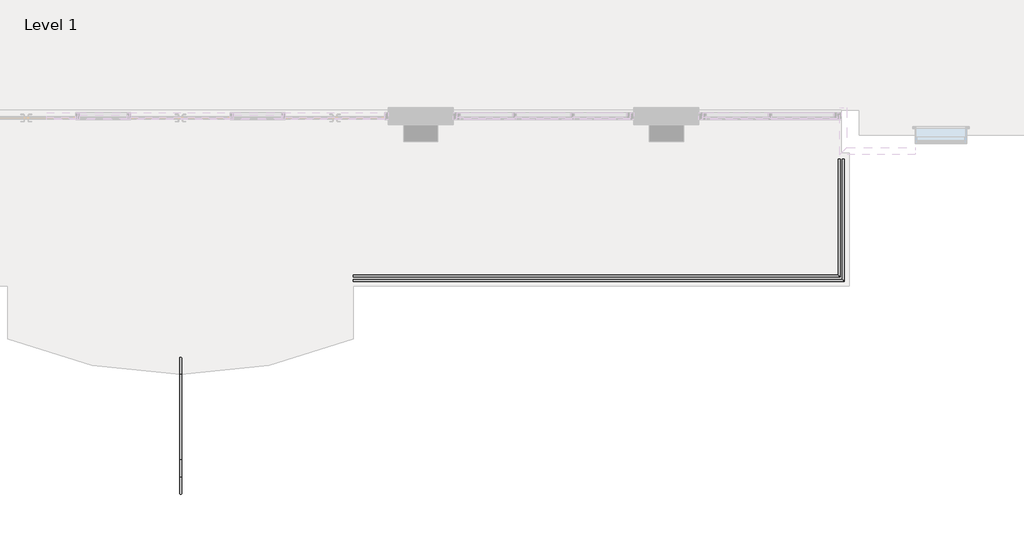
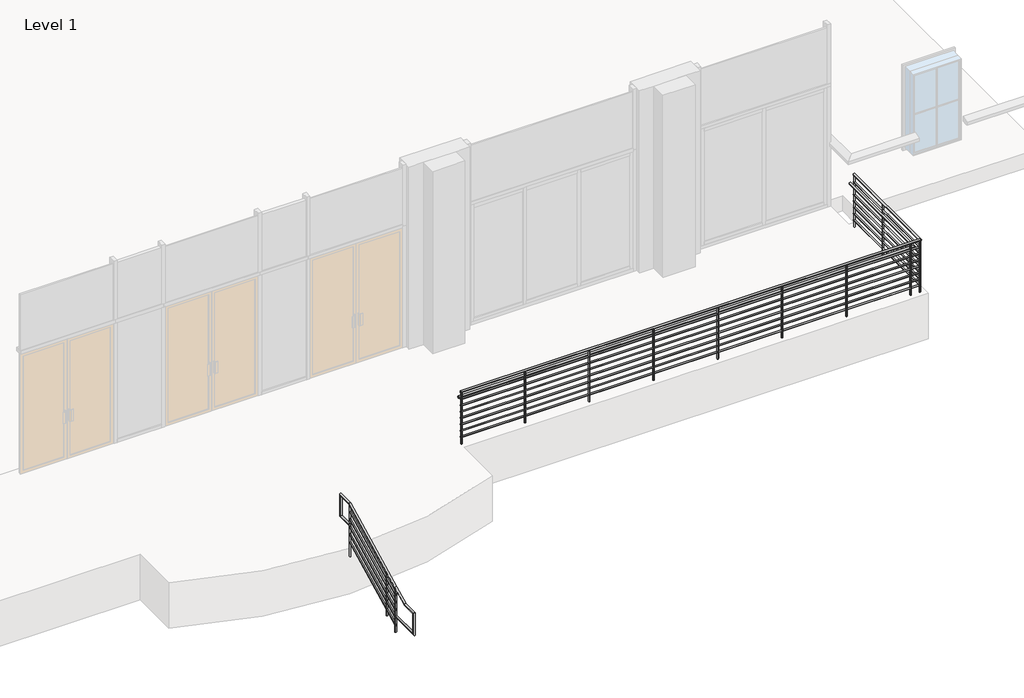
# One storey, part 3 of 5: 2 railings.
"""IFC4 building model written with IfcOpenShell, lengths in millimetres."""

import ifcopenshell
import ifcopenshell.guid

model = None  # the IFC model being written
_history = None  # IfcOwnerHistory: only IFC2X3 demands one
_inside = {}  # id of a spatial element -> (the spatial element, [elements in it])
_under = {}  # id of a project, library or spatial element -> (it, [spatial elements below it])
_declared = {}  # id of a project -> (the project, [libraries it declares])
_typed = {}  # id of a type object -> (the type object, [elements of that type])
_made_of = {}  # id of a material, layer set ... -> (it, [elements and type objects made of it])


def new_model(schema):
    """Start an empty IFC model of exactly this schema.

    Asked for "IFC4X3", IfcOpenShell would pick the latest addendum, in which some entities
    have other attributes; the version numbers below select the first issue.
    IFC2X3 requires an IfcOwnerHistory on every rooted entity: one is made here for all.
    """
    global model, _history
    if schema == "IFC4X3":
        model = ifcopenshell.file(schema_version=(4, 3, 0, 0))
    else:
        model = ifcopenshell.file(schema=schema)
    _inside.clear()
    _under.clear()
    _declared.clear()
    _typed.clear()
    _made_of.clear()
    _history = None
    if model.schema == "IFC2X3":
        org = make("IfcOrganization", Name="unknown")
        user = make(
            "IfcPersonAndOrganization",
            ThePerson=make("IfcPerson", FamilyName="unknown"),
            TheOrganization=org,
        )
        app = make(
            "IfcApplication",
            ApplicationDeveloper=org,
            Version="unknown",
            ApplicationFullName="unknown",
            ApplicationIdentifier="unknown",
        )
        _history = make(
            "IfcOwnerHistory",
            OwningUser=user,
            OwningApplication=app,
            ChangeAction="ADDED",
            CreationDate=0,
        )
    return model


def make(cls, **values):
    """One entity of the class cls with the attributes given. An attribute that is None is left unset."""
    return model.create_entity(
        cls, **{name: value for name, value in values.items() if value is not None}
    )


def rooted(cls, **values):
    """An entity with a GlobalId (a new one), such as an element, a storey or a relation."""
    return make(cls, GlobalId=ifcopenshell.guid.new(), OwnerHistory=_history, **values)


def si_unit(unit_type, name, prefix=None):
    """IfcSIUnit, for example si_unit("LENGTHUNIT", "METRE", prefix="MILLI")."""
    return make("IfcSIUnit", UnitType=unit_type, Prefix=prefix, Name=name)


def assignment(units):
    """IfcUnitAssignment: the units of a project."""
    return None if units is None else make("IfcUnitAssignment", Units=units)


def point(xyz):
    """IfcCartesianPoint."""
    return None if xyz is None else make("IfcCartesianPoint", Coordinates=xyz)


def direction(xyz):
    """IfcDirection."""
    return None if xyz is None else make("IfcDirection", DirectionRatios=xyz)


def frame(location, z_axis=None, x_axis=None):
    """IfcAxis2Placement3D, a coordinate frame: its origin and axes. An axis left out is left unset."""
    return make(
        "IfcAxis2Placement3D",
        Location=point(location),
        Axis=direction(z_axis),
        RefDirection=direction(x_axis),
    )


def frame_2d(location, x_axis=None):
    """IfcAxis2Placement2D, a coordinate frame in the plane: its origin and x axis."""
    return make(
        "IfcAxis2Placement2D", Location=point(location), RefDirection=direction(x_axis)
    )


def origin():
    """The frame at (0, 0, 0) with its axes left unset."""
    return frame((0.0, 0.0, 0.0))


def origin_with_axes():
    """The frame at (0, 0, 0) with the z axis (0, 0, 1) and the x axis (1, 0, 0) written out."""
    return frame((0.0, 0.0, 0.0), z_axis=(0.0, 0.0, 1.0), x_axis=(1.0, 0.0, 0.0))


def place(relative_to, where):
    """IfcLocalPlacement: puts the frame where relative to a parent placement (None: the world)."""
    return make(
        "IfcLocalPlacement", PlacementRelTo=relative_to, RelativePlacement=where
    )


def context(
    kind, dimensions, precision=None, world=None, true_north=None, identifier=None
):
    """IfcGeometricRepresentationContext, for example the 3D "Model" context."""
    return make(
        "IfcGeometricRepresentationContext",
        ContextIdentifier=identifier,
        ContextType=kind,
        CoordinateSpaceDimension=dimensions,
        Precision=precision,
        WorldCoordinateSystem=world,
        TrueNorth=true_north,
    )


def project(units=None, contexts=None):
    """IfcProject with its units and contexts."""
    return rooted(
        "IfcProject",
        Name="project",
        RepresentationContexts=contexts,
        UnitsInContext=assignment(units),
    )


def spatial(cls, under=None, at=None, **own):
    """A site, building, storey or space (cls), placed at a placement, below another one or the project."""
    s = rooted(cls, ObjectPlacement=at, **own)
    if under is not None:
        _under.setdefault(under.id(), (under, []))[1].append(s)
    return s


def circle_curve(where, radius):
    """IfcCircle in the frame where."""
    return make("IfcCircle", Position=where, Radius=radius)


def ellipse_curve(where, semi_axis1, semi_axis2):
    """IfcEllipse in the frame where."""
    return make(
        "IfcEllipse", Position=where, SemiAxis1=semi_axis1, SemiAxis2=semi_axis2
    )


def trimmed(basis, trim1, trim2, sense, master):
    """IfcTrimmedCurve: the piece of a basis curve between two trims."""
    return make(
        "IfcTrimmedCurve",
        BasisCurve=basis,
        Trim1=trim1,
        Trim2=trim2,
        SenseAgreement=sense,
        MasterRepresentation=master,
    )


def segment(curve, same_sense, transition):
    """IfcCompositeCurveSegment."""
    return make(
        "IfcCompositeCurveSegment",
        Transition=transition,
        SameSense=same_sense,
        ParentCurve=curve,
    )


def composite_curve(segments, self_intersect=None):
    """IfcCompositeCurve: segments joined end to end."""
    return make("IfcCompositeCurve", Segments=segments, SelfIntersect=self_intersect)


def outline(outer, holes=None, kind="AREA"):
    """IfcArbitraryClosedProfileDef: a profile drawn as a closed curve; with holes, ...WithVoids."""
    if holes is None:
        return make("IfcArbitraryClosedProfileDef", ProfileType=kind, OuterCurve=outer)
    return make(
        "IfcArbitraryProfileDefWithVoids",
        ProfileType=kind,
        OuterCurve=outer,
        InnerCurves=holes,
    )


def extrude(swept, where, along, depth):
    """IfcExtrudedAreaSolid: the profile swept, set in the frame where, extruded along a direction by depth."""
    return make(
        "IfcExtrudedAreaSolid",
        SweptArea=swept,
        Position=where,
        ExtrudedDirection=direction(along),
        Depth=depth,
    )


def shape(context_of_items, identifier, shape_type, items):
    """IfcShapeRepresentation: the items that make up one representation, for example the "Body"."""
    return make(
        "IfcShapeRepresentation",
        ContextOfItems=context_of_items,
        RepresentationIdentifier=identifier,
        RepresentationType=shape_type,
        Items=items,
    )


def made_of(thing, what):
    """Note that an element or type object is made of a material, layer set ...; save() writes the relation."""
    if what is not None:
        _made_of.setdefault(what.id(), (what, []))[1].append(thing)
    return thing


def element(
    cls,
    number,
    at=None,
    inside=None,
    cuts=None,
    type_object=None,
    material=None,
    context=None,
    identifier="Body",
    shape_type=None,
    held_by="IfcProductDefinitionShape",
    body=None,
    shapes=None,
    **own,
):
    """One element of the class cls, such as IfcWall. Its Tag is "e" and its number.

    at: its placement. inside: the storey or other place that contains it. cuts: it is an
    opening in that element (IfcRelVoidsElement). A single representation is given by context,
    identifier, shape_type and body (its items); several are given by shapes. held_by: the class
    of the entity that holds the representations. save() writes the other relations.
    """
    e = rooted(cls, Tag="e%d" % number, ObjectPlacement=at, **own)
    if body is not None:
        shapes = [shape(context, identifier, shape_type, body)]
    if shapes is not None:
        e.Representation = make(held_by, Representations=shapes)
    if inside is not None:
        _inside.setdefault(inside.id(), (inside, []))[1].append(e)
    if cuts is not None:
        rooted(
            "IfcRelVoidsElement", RelatingBuildingElement=cuts, RelatedOpeningElement=e
        )
    if type_object is not None:
        _typed.setdefault(type_object.id(), (type_object, []))[1].append(e)
    return made_of(e, material)


def aggregate(whole, parts):
    """IfcRelAggregates: a whole, such as a stair, and the parts it consists of."""
    return rooted("IfcRelAggregates", RelatingObject=whole, RelatedObjects=parts)


def save(model, path):
    """Write the relations noted so far, then the file.

    IfcRelAggregates (storeys below a building ...), IfcRelContainedInSpatialStructure (elements
    in a storey), IfcRelDefinesByType, IfcRelAssociatesMaterial and IfcRelDeclares: one each for
    every whole, place, type object, material and project.
    """
    for whole, parts in _under.values():
        aggregate(whole, parts)
    for where, things in _inside.values():
        rooted(
            "IfcRelContainedInSpatialStructure",
            RelatedElements=things,
            RelatingStructure=where,
        )
    for kind, things in _typed.values():
        rooted("IfcRelDefinesByType", RelatedObjects=things, RelatingType=kind)
    for what, things in _made_of.values():
        rooted("IfcRelAssociatesMaterial", RelatedObjects=things, RelatingMaterial=what)
    for by, libraries in _declared.values():
        rooted("IfcRelDeclares", RelatingContext=by, RelatedDefinitions=libraries)
    model.write(path)


def plane_surface(at):
    """IfcPlane: the flat surface through the origin of the frame at, square to its z axis."""
    return make("IfcPlane", Position=at)


def cylinder_surface(at, radius):
    """IfcCylindricalSurface: all points at the distance radius from the z axis of the frame at."""
    return make("IfcCylindricalSurface", Position=at, Radius=radius)


def advanced_brep(points, edges, surfaces, faces):
    """IfcAdvancedBrep: a solid bounded by faces that lie on surfaces and meet in shared edges.

    An edge is (start, end): straight between two places in points (the first is 0);
    or (start, end, curve); or (start, end, curve, False) where it runs against its curve.
    A face is (place in surfaces, loops), or (place, loops, False) where it looks against
    its surface's normal. A loop lists edges by number (the first is 1), with a minus sign
    where the edge is run from its end to its start. The first loop is the outer one.
    """
    corners = [point(p) for p in points]
    vertices = [make("IfcVertexPoint", VertexGeometry=c) for c in corners]
    made = []
    for start, end, *more in edges:
        made.append(
            make(
                "IfcEdgeCurve",
                EdgeStart=vertices[start],
                EdgeEnd=vertices[end],
                EdgeGeometry=more[0] if more else make("IfcPolyline", Points=[corners[start], corners[end]]),
                SameSense=more[1] if len(more) > 1 else True,
            )
        )
    hull = []
    for where, loops, *sense in faces:
        bounds = []
        for j, loop in enumerate(loops):
            ring = [make("IfcOrientedEdge", EdgeElement=made[abs(k) - 1], Orientation=k > 0) for k in loop]
            bounds.append(
                make(
                    "IfcFaceOuterBound" if j == 0 else "IfcFaceBound",
                    Bound=make("IfcEdgeLoop", EdgeList=ring),
                    Orientation=True,
                )
            )
        hull.append(make("IfcAdvancedFace", Bounds=bounds, FaceSurface=surfaces[where], SameSense=sense[0] if sense else True))
    return make("IfcAdvancedBrep", Outer=make("IfcClosedShell", CfsFaces=hull))


model = new_model("IFC4")

# Units and contexts
model_context = context("Model", 3, world=origin())
ifc_project = project(units=[si_unit("LENGTHUNIT", "METRE", prefix="MILLI")], contexts=[model_context])

# Site, building, storey
site = spatial("IfcSite", under=ifc_project)
building = spatial("IfcBuilding", under=site)
storey = spatial("IfcBuildingStorey", under=building, Name="Level 1", Elevation=0.0)

# Railings
placement = place(None, origin())
element("IfcRailing", 1, ObjectType="Handrail – Pipe – Bottom &Top Extension", at=placement, inside=storey, context=model_context, shape_type="AdvancedBrep", body=[
    advanced_brep(
    [(-1146.7622732, -15471.359437, -438.15), (-1184.8622732, -15471.359437, -438.15), (-1146.7622732, -16062.2278525, -438.15), (-1184.8622732, -16062.2278525, -438.15), (-1146.7622732, -16062.2278525, -19.05), (-1184.8622732, -16062.2278525, -19.05), (-1146.7622732, -15771.9807575, -19.05), (-1184.8622732, -15771.9807575, -19.05), (-1146.7622732, -15463.1584335, 135.361162), (-1184.8622732, -15463.1584335, 135.361162), (-1146.7622732, -13943.1807575, 895.35), (-1184.8622732, -13943.1807575, 895.35), (-1146.7622732, -13661.9278525, 895.35), (-1184.8622732, -13661.9278525, 895.35), (-1146.7622732, -13661.9278525, 476.25), (-1184.8622732, -13661.9278525, 476.25), (-1146.7622732, -13947.996268, 476.25), (-1184.8622732, -13947.996268, 476.25)],
    [
        (0, 1, circle_curve(frame((-1165.8122732, -15471.359437, -438.15), z_axis=(0.0, 1.0, 0.0), x_axis=(-1.0, 0.0, 0.0)), 19.05)),
        (1, 0, circle_curve(frame((-1165.8122732, -15471.359437, -438.15), z_axis=(0.0, 1.0, 0.0), x_axis=(-1.0, 0.0, 0.0)), 19.05)),
        (0, 2),
        (2, 3, ellipse_curve(frame((-1165.8122732, -16062.2278525, -438.15), z_axis=(0.0, 0.7071067811865475, -0.7071067811865475), x_axis=(0.0, 0.7071067811865476, 0.7071067811865474)), 26.9407684, 19.05)),
        (3, 1),
        (3, 2, ellipse_curve(frame((-1165.8122732, -16062.2278525, -438.15), z_axis=(0.0, 0.7071067811865475, -0.7071067811865475), x_axis=(0.0, 0.7071067811865476, 0.7071067811865474)), 26.9407684, 19.05)),
        (2, 4),
        (4, 5, ellipse_curve(frame((-1165.8122732, -16062.2278525, -19.05), z_axis=(0.0, -0.7071067811865475, -0.7071067811865475), x_axis=(0.0, 0.7071067811865474, -0.7071067811865476)), 26.9407684, 19.05)),
        (5, 3),
        (5, 4, ellipse_curve(frame((-1165.8122732, -16062.2278525, -19.05), z_axis=(0.0, -0.7071067811865475, -0.7071067811865475), x_axis=(0.0, 0.7071067811865474, -0.7071067811865476)), 26.9407684, 19.05)),
        (4, 6),
        (6, 7, ellipse_curve(frame((-1165.8122732, -15771.9807575, -19.05), z_axis=(0.0, -0.9732489894677302, -0.22975292054736124), x_axis=(0.0, -0.22975292054736096, 0.9732489894677302)), 19.573614, 19.05)),
        (7, 5),
        (7, 6, ellipse_curve(frame((-1165.8122732, -15771.9807575, -19.05), z_axis=(0.0, -0.9732489894677302, -0.22975292054736124), x_axis=(0.0, -0.22975292054736096, 0.9732489894677302)), 19.573614, 19.05)),
        (6, 8),
        (8, 9, circle_curve(frame((-1165.8122732, -15463.1584335, 135.361162), z_axis=(0.0, -0.8944271909999159, -0.44721359549995804), x_axis=(-1.0, 0.0, 0.0)), 19.05)),
        (9, 7),
        (9, 8, circle_curve(frame((-1165.8122732, -15463.1584335, 135.361162), z_axis=(0.0, -0.8944271909999159, -0.44721359549995804), x_axis=(-1.0, 0.0, 0.0)), 19.05)),
        (8, 10),
        (10, 11, ellipse_curve(frame((-1165.8122732, -13943.1807575, 895.35), z_axis=(0.0, -0.9732489894677302, -0.22975292054736132), x_axis=(0.0, 0.2297529205473615, -0.9732489894677301)), 19.573614, 19.05)),
        (11, 9),
        (11, 10, ellipse_curve(frame((-1165.8122732, -13943.1807575, 895.35), z_axis=(0.0, -0.9732489894677302, -0.22975292054736132), x_axis=(0.0, 0.2297529205473615, -0.9732489894677301)), 19.573614, 19.05)),
        (10, 12),
        (12, 13, ellipse_curve(frame((-1165.8122732, -13661.9278525, 895.35), z_axis=(0.0, -0.7071067811865476, 0.7071067811865474), x_axis=(0.0, -0.7071067811865475, -0.7071067811865475)), 26.9407684, 19.05)),
        (13, 11),
        (13, 12, ellipse_curve(frame((-1165.8122732, -13661.9278525, 895.35), z_axis=(0.0, -0.7071067811865476, 0.7071067811865474), x_axis=(0.0, -0.7071067811865475, -0.7071067811865475)), 26.9407684, 19.05)),
        (12, 14),
        (14, 15, ellipse_curve(frame((-1165.8122732, -13661.9278525, 476.25), z_axis=(0.0, 0.7071067811865474, 0.7071067811865476), x_axis=(0.0, -0.7071067811865475, 0.7071067811865475)), 26.9407684, 19.05)),
        (15, 13),
        (15, 14, ellipse_curve(frame((-1165.8122732, -13661.9278525, 476.25), z_axis=(0.0, 0.7071067811865474, 0.7071067811865476), x_axis=(0.0, -0.7071067811865475, 0.7071067811865475)), 26.9407684, 19.05)),
        (16, 17, circle_curve(frame((-1165.8122732, -13947.996268, 476.25), z_axis=(0.0, -1.0, 0.0), x_axis=(-1.0, 0.0, 0.0)), 19.05)),
        (17, 16, circle_curve(frame((-1165.8122732, -13947.996268, 476.25), z_axis=(0.0, -1.0, 0.0), x_axis=(-1.0, 0.0, 0.0)), 19.05)),
        (14, 16),
        (17, 15),
    ],
    [
        plane_surface(frame((-1165.8122732, -15471.359437, -457.2), z_axis=(0.0, 1.0, 0.0), x_axis=(0.0, 0.0, -1.0))),
        cylinder_surface(frame((-1165.8122732, -15471.359437, -438.15), z_axis=(0.0, 1.0, 0.0), x_axis=(-1.0, 0.0, 0.0)), 19.05),
        cylinder_surface(frame((-1165.8122732, -16062.2278525, -457.2), z_axis=(0.0, 0.0, -1.0), x_axis=(-1.0, 0.0, 0.0)), 19.05),
        cylinder_surface(frame((-1165.8122732, -16081.2778525, -19.05), z_axis=(0.0, -1.0, 0.0), x_axis=(-1.0, 0.0, 0.0)), 19.05),
        cylinder_surface(frame((-1165.8122732, -15767.9584335, -17.038838), z_axis=(0.0, -0.8944271909999159, -0.44721359549995804), x_axis=(-1.0, 0.0, 0.0)), 19.05),
        cylinder_surface(frame((-1165.8122732, -15463.1584335, 135.361162), z_axis=(0.0, -0.8944271909999159, -0.44721359549995804), x_axis=(-1.0, 0.0, 0.0)), 19.05),
        cylinder_surface(frame((-1165.8122732, -13947.6778525, 895.35), z_axis=(0.0, -1.0, 0.0), x_axis=(-1.0, 0.0, 0.0)), 19.05),
        cylinder_surface(frame((-1165.8122732, -13661.9278525, 914.4), z_axis=(0.0, 0.0, 1.0), x_axis=(-1.0, 0.0, 0.0)), 19.05),
        plane_surface(frame((-1165.8122732, -13947.996268, 457.2), z_axis=(0.0, -1.0, 0.0), x_axis=(0.0, 0.0, -1.0))),
        cylinder_surface(frame((-1165.8122732, -13642.8778525, 476.25), z_axis=(0.0, 1.0, 0.0), x_axis=(-1.0, 0.0, 0.0)), 19.05),
    ],
    [
        (0, [[1, 2]]),
        (1, [[-1, 3, 4, 5]]),
        (1, [[-2, -5, 6, -3]]),
        (2, [[-4, 7, 8, 9]]),
        (2, [[-6, -9, 10, -7]]),
        (3, [[-8, 11, 12, 13]]),
        (3, [[-10, -13, 14, -11]]),
        (4, [[-12, 15, 16, 17]]),
        (4, [[-14, -17, 18, -15]]),
        (5, [[-16, 19, 20, 21]]),
        (5, [[-18, -21, 22, -19]]),
        (6, [[-20, 23, 24, 25]]),
        (6, [[-22, -25, 26, -23]]),
        (7, [[-24, 27, 28, 29]]),
        (7, [[-26, -29, 30, -27]]),
        (8, [[31, 32]]),
        (9, [[-28, 33, -32, 34]]),
        (9, [[-30, -34, -31, -33]]),
    ],
),
    advanced_brep(
    [(-1153.1122732, -13947.6778525, 747.8009683), (-1178.5122732, -13947.6778525, 747.8009683), (-1153.1122732, -15471.6778525, -14.1990317), (-1178.5122732, -15471.6778525, -14.1990317)],
    [
        (0, 1, ellipse_curve(frame((-1165.8122732, -13947.6778525, 747.8009683), z_axis=(0.0, 1.0, 0.0), x_axis=(0.0, 0.0, 1.0)), 14.1990317, 12.7)),
        (1, 0, ellipse_curve(frame((-1165.8122732, -13947.6778525, 747.8009683), z_axis=(0.0, 1.0, 0.0), x_axis=(0.0, 0.0, 1.0)), 14.1990317, 12.7)),
        (2, 3, ellipse_curve(frame((-1165.8122732, -15471.6778525, -14.1990317), z_axis=(0.0, -1.0, 0.0), x_axis=(0.0, 0.0, 1.0)), 14.1990317, 12.7)),
        (3, 2, ellipse_curve(frame((-1165.8122732, -15471.6778525, -14.1990317), z_axis=(0.0, -1.0, 0.0), x_axis=(0.0, 0.0, 1.0)), 14.1990317, 12.7)),
        (0, 2),
        (3, 1),
    ],
    [
        plane_surface(frame((-1165.8122732, -13947.6778525, 762.0), z_axis=(0.0, 1.0, 0.0), x_axis=(0.0, 0.0, -1.0))),
        plane_surface(frame((-1165.8122732, -15471.6778525, 0.0), z_axis=(0.0, -1.0, 0.0), x_axis=(0.0, 0.0, -1.0))),
        cylinder_surface(frame((-1165.8122732, -13941.9982398, 750.6407747), z_axis=(0.0, 0.894427190999916, 0.447213595499958), x_axis=(-1.0, 0.0, 0.0)), 12.7),
    ],
    [
        (0, [[1, 2]]),
        (1, [[3, 4]]),
        (2, [[-1, 5, -4, 6]]),
        (2, [[-2, -6, -3, -5]]),
    ],
),
    advanced_brep(
    [(-1153.1122732, -13947.6778525, 595.4009683), (-1178.5122732, -13947.6778525, 595.4009683), (-1153.1122732, -15471.6778525, -166.5990317), (-1178.5122732, -15471.6778525, -166.5990317)],
    [
        (0, 1, ellipse_curve(frame((-1165.8122732, -13947.6778525, 595.4009683), z_axis=(0.0, 1.0, 0.0), x_axis=(0.0, 0.0, 1.0)), 14.1990317, 12.7)),
        (1, 0, ellipse_curve(frame((-1165.8122732, -13947.6778525, 595.4009683), z_axis=(0.0, 1.0, 0.0), x_axis=(0.0, 0.0, 1.0)), 14.1990317, 12.7)),
        (2, 3, ellipse_curve(frame((-1165.8122732, -15471.6778525, -166.5990317), z_axis=(0.0, -1.0, 0.0), x_axis=(0.0, 0.0, 1.0)), 14.1990317, 12.7)),
        (3, 2, ellipse_curve(frame((-1165.8122732, -15471.6778525, -166.5990317), z_axis=(0.0, -1.0, 0.0), x_axis=(0.0, 0.0, 1.0)), 14.1990317, 12.7)),
        (0, 2),
        (3, 1),
    ],
    [
        plane_surface(frame((-1165.8122732, -13947.6778525, 609.6), z_axis=(0.0, 1.0, 0.0), x_axis=(0.0, 0.0, -1.0))),
        plane_surface(frame((-1165.8122732, -15471.6778525, -152.4), z_axis=(0.0, -1.0, 0.0), x_axis=(0.0, 0.0, -1.0))),
        cylinder_surface(frame((-1165.8122732, -13941.9982398, 598.2407747), z_axis=(0.0, 0.894427190999916, 0.447213595499958), x_axis=(-1.0, 0.0, 0.0)), 12.7),
    ],
    [
        (0, [[1, 2]]),
        (1, [[3, 4]]),
        (2, [[-1, 5, -4, 6]]),
        (2, [[-2, -6, -3, -5]]),
    ],
),
    advanced_brep(
    [(-1153.1122732, -13947.6778525, 443.0009683), (-1178.5122732, -13947.6778525, 443.0009683), (-1153.1122732, -15471.6778525, -318.9990317), (-1178.5122732, -15471.6778525, -318.9990317)],
    [
        (0, 1, ellipse_curve(frame((-1165.8122732, -13947.6778525, 443.0009683), z_axis=(0.0, 1.0, 0.0), x_axis=(0.0, 0.0, 1.0)), 14.1990317, 12.7)),
        (1, 0, ellipse_curve(frame((-1165.8122732, -13947.6778525, 443.0009683), z_axis=(0.0, 1.0, 0.0), x_axis=(0.0, 0.0, 1.0)), 14.1990317, 12.7)),
        (2, 3, ellipse_curve(frame((-1165.8122732, -15471.6778525, -318.9990317), z_axis=(0.0, -1.0, 0.0), x_axis=(0.0, 0.0, 1.0)), 14.1990317, 12.7)),
        (3, 2, ellipse_curve(frame((-1165.8122732, -15471.6778525, -318.9990317), z_axis=(0.0, -1.0, 0.0), x_axis=(0.0, 0.0, 1.0)), 14.1990317, 12.7)),
        (0, 2),
        (3, 1),
    ],
    [
        plane_surface(frame((-1165.8122732, -13947.6778525, 457.2), z_axis=(0.0, 1.0, 0.0), x_axis=(0.0, 0.0, -1.0))),
        plane_surface(frame((-1165.8122732, -15471.6778525, -304.8), z_axis=(0.0, -1.0, 0.0), x_axis=(0.0, 0.0, -1.0))),
        cylinder_surface(frame((-1165.8122732, -13941.9982398, 445.8407747), z_axis=(0.0, 0.894427190999916, 0.447213595499958), x_axis=(-1.0, 0.0, 0.0)), 12.7),
    ],
    [
        (0, [[1, 2]]),
        (1, [[3, 4]]),
        (2, [[-1, 5, -4, 6]]),
        (2, [[-2, -6, -3, -5]]),
    ],
),
    advanced_brep(
    [(-1153.1122732, -13947.6778525, 290.6009683), (-1178.5122732, -13947.6778525, 290.6009683), (-1153.1122732, -15471.6778525, -471.3990317), (-1178.5122732, -15471.6778525, -471.3990317)],
    [
        (0, 1, ellipse_curve(frame((-1165.8122732, -13947.6778525, 290.6009683), z_axis=(0.0, 1.0, 0.0), x_axis=(0.0, 0.0, 1.0)), 14.1990317, 12.7)),
        (1, 0, ellipse_curve(frame((-1165.8122732, -13947.6778525, 290.6009683), z_axis=(0.0, 1.0, 0.0), x_axis=(0.0, 0.0, 1.0)), 14.1990317, 12.7)),
        (2, 3, ellipse_curve(frame((-1165.8122732, -15471.6778525, -471.3990317), z_axis=(0.0, -1.0, 0.0), x_axis=(0.0, 0.0, 1.0)), 14.1990317, 12.7)),
        (3, 2, ellipse_curve(frame((-1165.8122732, -15471.6778525, -471.3990317), z_axis=(0.0, -1.0, 0.0), x_axis=(0.0, 0.0, 1.0)), 14.1990317, 12.7)),
        (0, 2),
        (3, 1),
    ],
    [
        plane_surface(frame((-1165.8122732, -13947.6778525, 304.8), z_axis=(0.0, 1.0, 0.0), x_axis=(0.0, 0.0, -1.0))),
        plane_surface(frame((-1165.8122732, -15471.6778525, -457.2), z_axis=(0.0, -1.0, 0.0), x_axis=(0.0, 0.0, -1.0))),
        cylinder_surface(frame((-1165.8122732, -13941.9982398, 293.4407747), z_axis=(0.0, 0.894427190999916, 0.447213595499958), x_axis=(-1.0, 0.0, 0.0)), 12.7),
    ],
    [
        (0, [[1, 2]]),
        (1, [[3, 4]]),
        (2, [[-1, 5, -4, 6]]),
        (2, [[-2, -6, -3, -5]]),
    ],
),
    advanced_brep(
    [(-1153.1122732, -13947.6778525, 138.2009683), (-1178.5122732, -13947.6778525, 138.2009683), (-1153.1122732, -15471.6778525, -623.7990317), (-1178.5122732, -15471.6778525, -623.7990317)],
    [
        (0, 1, ellipse_curve(frame((-1165.8122732, -13947.6778525, 138.2009683), z_axis=(0.0, 1.0, 0.0), x_axis=(0.0, 0.0, 1.0)), 14.1990317, 12.7)),
        (1, 0, ellipse_curve(frame((-1165.8122732, -13947.6778525, 138.2009683), z_axis=(0.0, 1.0, 0.0), x_axis=(0.0, 0.0, 1.0)), 14.1990317, 12.7)),
        (2, 3, ellipse_curve(frame((-1165.8122732, -15471.6778525, -623.7990317), z_axis=(0.0, -1.0, 0.0), x_axis=(0.0, 0.0, 1.0)), 14.1990317, 12.7)),
        (3, 2, ellipse_curve(frame((-1165.8122732, -15471.6778525, -623.7990317), z_axis=(0.0, -1.0, 0.0), x_axis=(0.0, 0.0, 1.0)), 14.1990317, 12.7)),
        (0, 2),
        (3, 1),
    ],
    [
        plane_surface(frame((-1165.8122732, -13947.6778525, 152.4), z_axis=(0.0, 1.0, 0.0), x_axis=(0.0, 0.0, -1.0))),
        plane_surface(frame((-1165.8122732, -15471.6778525, -609.6), z_axis=(0.0, -1.0, 0.0), x_axis=(0.0, 0.0, -1.0))),
        cylinder_surface(frame((-1165.8122732, -13941.9982398, 141.0407747), z_axis=(0.0, 0.894427190999916, 0.447213595499958), x_axis=(-1.0, 0.0, 0.0)), 12.7),
    ],
    [
        (0, [[1, 2]]),
        (1, [[3, 4]]),
        (2, [[-1, 5, -4, 6]]),
        (2, [[-2, -6, -3, -5]]),
    ],
),
    advanced_brep(
    [(-1178.5122732, -15166.8778525, 262.202905), (-1178.5122732, -15166.8778525, -609.6), (-1153.1122732, -15166.8778525, -609.6), (-1153.1122732, -15166.8778525, 262.202905)],
    [
        (0, 1),
        (1, 2, circle_curve(frame((-1165.8122732, -15166.8778525, -609.6), z_axis=(0.0, 0.0, 1.0), x_axis=(1.0, 0.0, 0.0)), 12.7)),
        (2, 3),
        (3, 0, ellipse_curve(frame((-1165.8122732, -15166.8778525, 262.202905), z_axis=(0.0, 0.4472135954999566, -0.8944271909999165), x_axis=(0.0, 0.8944271909999165, 0.4472135954999567)), 14.1990317, 12.7)),
        (0, 3, ellipse_curve(frame((-1165.8122732, -15166.8778525, 262.202905), z_axis=(0.0, 0.4472135954999566, -0.8944271909999165), x_axis=(0.0, 0.8944271909999165, 0.4472135954999567)), 14.1990317, 12.7)),
        (2, 1, circle_curve(frame((-1165.8122732, -15166.8778525, -609.6), z_axis=(0.0, 0.0, 1.0), x_axis=(1.0, 0.0, 0.0)), 12.7)),
    ],
    [
        cylinder_surface(frame((-1165.8122732, -15166.8778525, -838.2), z_axis=(0.0, 0.0, 1.0), x_axis=(1.0, 0.0, 0.0)), 12.7),
        plane_surface(frame((-1140.4122732, -15192.2778525, 249.502905), z_axis=(0.0, -0.4472135954999566, 0.8944271909999165), x_axis=(-1.0, 0.0, 0.0))),
        plane_surface(frame((-1140.4122732, -15141.4778525, -609.6), z_axis=(0.0, 0.0, -1.0), x_axis=(-1.0, 0.0, 0.0))),
    ],
    [
        (0, [[1, 2, 3, 4]]),
        (0, [[-1, 5, -3, 6]]),
        (1, [[-4, -5]]),
        (2, [[-2, -6]]),
    ],
),
    advanced_brep(
    [(-1178.5122732, -15458.9778525, 116.152905), (-1178.5122732, -15458.9778525, -762.0), (-1153.1122732, -15458.9778525, -762.0), (-1153.1122732, -15458.9778525, 116.152905)],
    [
        (0, 1),
        (1, 2, circle_curve(frame((-1165.8122732, -15458.9778525, -762.0), z_axis=(0.0, 0.0, 1.0), x_axis=(1.0, 0.0, 0.0)), 12.7)),
        (2, 3),
        (3, 0, ellipse_curve(frame((-1165.8122732, -15458.9778525, 116.152905), z_axis=(0.0, 0.4472135954999566, -0.8944271909999165), x_axis=(0.0, 0.8944271909999165, 0.4472135954999567)), 14.1990317, 12.7)),
        (0, 3, ellipse_curve(frame((-1165.8122732, -15458.9778525, 116.152905), z_axis=(0.0, 0.4472135954999566, -0.8944271909999165), x_axis=(0.0, 0.8944271909999165, 0.4472135954999567)), 14.1990317, 12.7)),
        (2, 1, circle_curve(frame((-1165.8122732, -15458.9778525, -762.0), z_axis=(0.0, 0.0, 1.0), x_axis=(1.0, 0.0, 0.0)), 12.7)),
    ],
    [
        cylinder_surface(frame((-1165.8122732, -15458.9778525, -990.6), z_axis=(0.0, 0.0, 1.0), x_axis=(1.0, 0.0, 0.0)), 12.7),
        plane_surface(frame((-1140.4122732, -15484.3778525, 103.452905), z_axis=(0.0, -0.4472135954999566, 0.8944271909999165), x_axis=(-1.0, 0.0, 0.0))),
        plane_surface(frame((-1140.4122732, -15433.5778525, -762.0), z_axis=(0.0, 0.0, -1.0), x_axis=(-1.0, 0.0, 0.0))),
    ],
    [
        (0, [[1, 2, 3, 4]]),
        (0, [[-1, 5, -3, 6]]),
        (1, [[-4, -5]]),
        (2, [[-2, -6]]),
    ],
),
    advanced_brep(
    [(-1178.5122732, -13960.3778525, 865.452905), (-1178.5122732, -13960.3778525, -152.4), (-1153.1122732, -13960.3778525, -152.4), (-1153.1122732, -13960.3778525, 865.452905)],
    [
        (0, 1),
        (1, 2, circle_curve(frame((-1165.8122732, -13960.3778525, -152.4), z_axis=(0.0, 0.0, 1.0), x_axis=(1.0, 0.0, 0.0)), 12.7)),
        (2, 3),
        (3, 0, ellipse_curve(frame((-1165.8122732, -13960.3778525, 865.452905), z_axis=(0.0, 0.4472135954999566, -0.8944271909999165), x_axis=(0.0, 0.8944271909999165, 0.4472135954999567)), 14.1990317, 12.7)),
        (0, 3, ellipse_curve(frame((-1165.8122732, -13960.3778525, 865.452905), z_axis=(0.0, 0.4472135954999566, -0.8944271909999165), x_axis=(0.0, 0.8944271909999165, 0.4472135954999567)), 14.1990317, 12.7)),
        (2, 1, circle_curve(frame((-1165.8122732, -13960.3778525, -152.4), z_axis=(0.0, 0.0, 1.0), x_axis=(1.0, 0.0, 0.0)), 12.7)),
    ],
    [
        cylinder_surface(frame((-1165.8122732, -13960.3778525, -381.0), z_axis=(0.0, 0.0, 1.0), x_axis=(1.0, 0.0, 0.0)), 12.7),
        plane_surface(frame((-1140.4122732, -13985.7778525, 852.752905), z_axis=(0.0, -0.4472135954999566, 0.8944271909999165), x_axis=(-1.0, 0.0, 0.0))),
        plane_surface(frame((-1140.4122732, -13934.9778525, -152.4), z_axis=(0.0, 0.0, -1.0), x_axis=(-1.0, 0.0, 0.0))),
    ],
    [
        (0, [[1, 2, 3, 4]]),
        (0, [[-1, 5, -3, 6]]),
        (1, [[-4, -5]]),
        (2, [[-2, -6]]),
    ],
),
])
element("IfcRailing", 2, ObjectType="Guardrail - Pipe", at=placement, inside=storey, context=model_context, shape_type="SolidModel", body=[
    advanced_brep(
    [(1903.9547354, -12217.7608439, 895.35), (1903.9547354, -12179.6608439, 895.35), (10558.224655, -12217.7608439, 895.35), (10520.124655, -12179.6608439, 895.35), (10558.224655, -10114.0984696, 895.35), (10520.124655, -10114.0984696, 895.35)],
    [
        (0, 1, circle_curve(frame((1903.9547354, -12198.7108439, 895.35), z_axis=(-1.0, 0.0, 0.0), x_axis=(0.0, 1.0, 0.0)), 19.05)),
        (1, 0, circle_curve(frame((1903.9547354, -12198.7108439, 895.35), z_axis=(-1.0, 0.0, 0.0), x_axis=(0.0, 1.0, 0.0)), 19.05)),
        (0, 2),
        (2, 3, ellipse_curve(frame((10539.174655, -12198.7108439, 895.35), z_axis=(-0.7071067811865475, -0.7071067811865475, 0.0), x_axis=(-0.7071067811865476, 0.7071067811865474, 0.0)), 26.9407684, 19.05)),
        (3, 1),
        (3, 2, ellipse_curve(frame((10539.174655, -12198.7108439, 895.35), z_axis=(-0.7071067811865475, -0.7071067811865475, 0.0), x_axis=(-0.7071067811865476, 0.7071067811865474, 0.0)), 26.9407684, 19.05)),
        (4, 5, circle_curve(frame((10539.174655, -10114.0984696, 895.35), z_axis=(0.0, 1.0, 0.0), x_axis=(-1.0, 0.0, 0.0)), 19.05)),
        (5, 4, circle_curve(frame((10539.174655, -10114.0984696, 895.35), z_axis=(0.0, 1.0, 0.0), x_axis=(-1.0, 0.0, 0.0)), 19.05)),
        (2, 4),
        (5, 3),
    ],
    [
        plane_surface(frame((1903.9547354, -12198.7108439, 914.4), z_axis=(-1.0, 0.0, 0.0), x_axis=(0.0, 1.0, 0.0))),
        cylinder_surface(frame((1903.9547354, -12198.7108439, 895.35), z_axis=(-1.0, 0.0, 0.0), x_axis=(0.0, 1.0, 0.0)), 19.05),
        plane_surface(frame((10539.174655, -10114.0984696, 914.4), z_axis=(0.0, 1.0, 0.0), x_axis=(0.0, 0.0, 1.0))),
        cylinder_surface(frame((10539.174655, -12198.7108439, 895.35), z_axis=(0.0, -1.0, 0.0), x_axis=(-1.0, 0.0, 0.0)), 19.05),
    ],
    [
        (0, [[1, 2]]),
        (1, [[-1, 3, 4, 5]]),
        (1, [[-2, -5, 6, -3]]),
        (2, [[7, 8]]),
        (3, [[-4, 9, -8, 10]]),
        (3, [[-6, -10, -7, -9]]),
    ],
),
    advanced_brep(
    [(1903.9547354, -12293.9608439, 1047.75), (1903.9547354, -12255.8608439, 1047.75), (10634.424655, -12293.9608439, 1047.75), (10596.324655, -12255.8608439, 1047.75), (10634.424655, -10114.0984696, 1047.75), (10596.324655, -10114.0984696, 1047.75)],
    [
        (0, 1, circle_curve(frame((1903.9547354, -12274.9108439, 1047.75), z_axis=(-1.0, 0.0, 0.0), x_axis=(0.0, 1.0, 0.0)), 19.05)),
        (1, 0, circle_curve(frame((1903.9547354, -12274.9108439, 1047.75), z_axis=(-1.0, 0.0, 0.0), x_axis=(0.0, 1.0, 0.0)), 19.05)),
        (0, 2),
        (2, 3, ellipse_curve(frame((10615.374655, -12274.9108439, 1047.75), z_axis=(-0.7071067811865475, -0.7071067811865475, 0.0), x_axis=(-0.7071067811865476, 0.7071067811865474, 0.0)), 26.9407684, 19.05)),
        (3, 1),
        (3, 2, ellipse_curve(frame((10615.374655, -12274.9108439, 1047.75), z_axis=(-0.7071067811865475, -0.7071067811865475, 0.0), x_axis=(-0.7071067811865476, 0.7071067811865474, 0.0)), 26.9407684, 19.05)),
        (4, 5, circle_curve(frame((10615.374655, -10114.0984696, 1047.75), z_axis=(0.0, 1.0, 0.0), x_axis=(-1.0, 0.0, 0.0)), 19.05)),
        (5, 4, circle_curve(frame((10615.374655, -10114.0984696, 1047.75), z_axis=(0.0, 1.0, 0.0), x_axis=(-1.0, 0.0, 0.0)), 19.05)),
        (2, 4),
        (5, 3),
    ],
    [
        plane_surface(frame((1903.9547354, -12274.9108439, 1066.8), z_axis=(-1.0, 0.0, 0.0), x_axis=(0.0, 1.0, 0.0))),
        cylinder_surface(frame((1903.9547354, -12274.9108439, 1047.75), z_axis=(-1.0, 0.0, 0.0), x_axis=(0.0, 1.0, 0.0)), 19.05),
        plane_surface(frame((10615.374655, -10114.0984696, 1066.8), z_axis=(0.0, 1.0, 0.0), x_axis=(0.0, 0.0, 1.0))),
        cylinder_surface(frame((10615.374655, -12274.9108439, 1047.75), z_axis=(0.0, -1.0, 0.0), x_axis=(-1.0, 0.0, 0.0)), 19.05),
    ],
    [
        (0, [[1, 2]]),
        (1, [[-1, 3, 4, 5]]),
        (1, [[-2, -5, 6, -3]]),
        (2, [[7, 8]]),
        (3, [[-4, 9, -8, 10]]),
        (3, [[-6, -10, -7, -9]]),
    ],
),
    extrude(outline(composite_curve([segment(trimmed(circle_curve(frame_2d((-12274.9108439, 901.7)), 12.7), [point((-12262.2108439, 901.7))], [point((-12287.6108439, 901.7))], False, "CARTESIAN"), True, "CONTINUOUS"), segment(trimmed(circle_curve(frame_2d((-12274.9108439, 901.7)), 12.7), [point((-12287.6108439, 901.7))], [point((-12262.2108439, 901.7))], False, "CARTESIAN"), True, "CONTINUOUS")], self_intersect=False)), frame((1903.9547354, 0.0, 0.0), z_axis=(1.0, 0.0, 0.0), x_axis=(0.0, 1.0, 0.0)), (0.0, 0.0, 1.0), 8698.7199196),
    extrude(outline(composite_curve([segment(trimmed(circle_curve(frame_2d((901.7, 10615.374655)), 12.7), [point((901.7, 10602.674655))], [point((901.7, 10628.074655))], False, "CARTESIAN"), True, "CONTINUOUS"), segment(trimmed(circle_curve(frame_2d((901.7, 10615.374655)), 12.7), [point((901.7, 10628.074655))], [point((901.7, 10602.674655))], False, "CARTESIAN"), True, "CONTINUOUS")], self_intersect=False)), frame((0.0, -12287.6108439, 0.0), z_axis=(0.0, 1.0, 0.0), x_axis=(0.0, 0.0, 1.0)), (0.0, 0.0, 1.0), 2173.5123743),
    extrude(outline(composite_curve([segment(trimmed(circle_curve(frame_2d((-12274.9108439, 774.7)), 12.7), [point((-12262.2108439, 774.7))], [point((-12287.6108439, 774.7))], False, "CARTESIAN"), True, "CONTINUOUS"), segment(trimmed(circle_curve(frame_2d((-12274.9108439, 774.7)), 12.7), [point((-12287.6108439, 774.7))], [point((-12262.2108439, 774.7))], False, "CARTESIAN"), True, "CONTINUOUS")], self_intersect=False)), frame((1903.9547354, 0.0, 0.0), z_axis=(1.0, 0.0, 0.0), x_axis=(0.0, 1.0, 0.0)), (0.0, 0.0, 1.0), 8698.7199196),
    extrude(outline(composite_curve([segment(trimmed(circle_curve(frame_2d((774.7, 10615.374655)), 12.7), [point((774.7, 10602.674655))], [point((774.7, 10628.074655))], False, "CARTESIAN"), True, "CONTINUOUS"), segment(trimmed(circle_curve(frame_2d((774.7, 10615.374655)), 12.7), [point((774.7, 10628.074655))], [point((774.7, 10602.674655))], False, "CARTESIAN"), True, "CONTINUOUS")], self_intersect=False)), frame((0.0, -12287.6108439, 0.0), z_axis=(0.0, 1.0, 0.0), x_axis=(0.0, 0.0, 1.0)), (0.0, 0.0, 1.0), 2173.5123743),
    extrude(outline(composite_curve([segment(trimmed(circle_curve(frame_2d((-12274.9108439, 647.7)), 12.7), [point((-12262.2108439, 647.7))], [point((-12287.6108439, 647.7))], False, "CARTESIAN"), True, "CONTINUOUS"), segment(trimmed(circle_curve(frame_2d((-12274.9108439, 647.7)), 12.7), [point((-12287.6108439, 647.7))], [point((-12262.2108439, 647.7))], False, "CARTESIAN"), True, "CONTINUOUS")], self_intersect=False)), frame((1903.9547354, 0.0, 0.0), z_axis=(1.0, 0.0, 0.0), x_axis=(0.0, 1.0, 0.0)), (0.0, 0.0, 1.0), 8698.7199196),
    extrude(outline(composite_curve([segment(trimmed(circle_curve(frame_2d((647.7, 10615.374655)), 12.7), [point((647.7, 10602.674655))], [point((647.7, 10628.074655))], False, "CARTESIAN"), True, "CONTINUOUS"), segment(trimmed(circle_curve(frame_2d((647.7, 10615.374655)), 12.7), [point((647.7, 10628.074655))], [point((647.7, 10602.674655))], False, "CARTESIAN"), True, "CONTINUOUS")], self_intersect=False)), frame((0.0, -12287.6108439, 0.0), z_axis=(0.0, 1.0, 0.0), x_axis=(0.0, 0.0, 1.0)), (0.0, 0.0, 1.0), 2173.5123743),
    extrude(outline(composite_curve([segment(trimmed(circle_curve(frame_2d((-12274.9108439, 520.7)), 12.7), [point((-12262.2108439, 520.7))], [point((-12287.6108439, 520.7))], False, "CARTESIAN"), True, "CONTINUOUS"), segment(trimmed(circle_curve(frame_2d((-12274.9108439, 520.7)), 12.7), [point((-12287.6108439, 520.7))], [point((-12262.2108439, 520.7))], False, "CARTESIAN"), True, "CONTINUOUS")], self_intersect=False)), frame((1903.9547354, 0.0, 0.0), z_axis=(1.0, 0.0, 0.0), x_axis=(0.0, 1.0, 0.0)), (0.0, 0.0, 1.0), 8698.7199196),
    extrude(outline(composite_curve([segment(trimmed(circle_curve(frame_2d((520.7, 10615.374655)), 12.7), [point((520.7, 10602.674655))], [point((520.7, 10628.074655))], False, "CARTESIAN"), True, "CONTINUOUS"), segment(trimmed(circle_curve(frame_2d((520.7, 10615.374655)), 12.7), [point((520.7, 10628.074655))], [point((520.7, 10602.674655))], False, "CARTESIAN"), True, "CONTINUOUS")], self_intersect=False)), frame((0.0, -12287.6108439, 0.0), z_axis=(0.0, 1.0, 0.0), x_axis=(0.0, 0.0, 1.0)), (0.0, 0.0, 1.0), 2173.5123743),
    extrude(outline(composite_curve([segment(trimmed(circle_curve(frame_2d((-12274.9108439, 393.7)), 12.7), [point((-12262.2108439, 393.7))], [point((-12287.6108439, 393.7))], False, "CARTESIAN"), True, "CONTINUOUS"), segment(trimmed(circle_curve(frame_2d((-12274.9108439, 393.7)), 12.7), [point((-12287.6108439, 393.7))], [point((-12262.2108439, 393.7))], False, "CARTESIAN"), True, "CONTINUOUS")], self_intersect=False)), frame((1903.9547354, 0.0, 0.0), z_axis=(1.0, 0.0, 0.0), x_axis=(0.0, 1.0, 0.0)), (0.0, 0.0, 1.0), 8698.7199196),
    extrude(outline(composite_curve([segment(trimmed(circle_curve(frame_2d((393.7, 10615.374655)), 12.7), [point((393.7, 10602.674655))], [point((393.7, 10628.074655))], False, "CARTESIAN"), True, "CONTINUOUS"), segment(trimmed(circle_curve(frame_2d((393.7, 10615.374655)), 12.7), [point((393.7, 10628.074655))], [point((393.7, 10602.674655))], False, "CARTESIAN"), True, "CONTINUOUS")], self_intersect=False)), frame((0.0, -12287.6108439, 0.0), z_axis=(0.0, 1.0, 0.0), x_axis=(0.0, 0.0, 1.0)), (0.0, 0.0, 1.0), 2173.5123743),
    extrude(outline(composite_curve([segment(trimmed(circle_curve(frame_2d((-12274.9108439, 266.7)), 12.7), [point((-12262.2108439, 266.7))], [point((-12287.6108439, 266.7))], False, "CARTESIAN"), True, "CONTINUOUS"), segment(trimmed(circle_curve(frame_2d((-12274.9108439, 266.7)), 12.7), [point((-12287.6108439, 266.7))], [point((-12262.2108439, 266.7))], False, "CARTESIAN"), True, "CONTINUOUS")], self_intersect=False)), frame((1903.9547354, 0.0, 0.0), z_axis=(1.0, 0.0, 0.0), x_axis=(0.0, 1.0, 0.0)), (0.0, 0.0, 1.0), 8698.7199196),
    extrude(outline(composite_curve([segment(trimmed(circle_curve(frame_2d((266.7, 10615.374655)), 12.7), [point((266.7, 10602.674655))], [point((266.7, 10628.074655))], False, "CARTESIAN"), True, "CONTINUOUS"), segment(trimmed(circle_curve(frame_2d((266.7, 10615.374655)), 12.7), [point((266.7, 10628.074655))], [point((266.7, 10602.674655))], False, "CARTESIAN"), True, "CONTINUOUS")], self_intersect=False)), frame((0.0, -12287.6108439, 0.0), z_axis=(0.0, 1.0, 0.0), x_axis=(0.0, 0.0, 1.0)), (0.0, 0.0, 1.0), 2173.5123743),
    extrude(outline(composite_curve([segment(trimmed(circle_curve(frame_2d((-12274.9108439, 139.7)), 12.7), [point((-12262.2108439, 139.7))], [point((-12287.6108439, 139.7))], False, "CARTESIAN"), True, "CONTINUOUS"), segment(trimmed(circle_curve(frame_2d((-12274.9108439, 139.7)), 12.7), [point((-12287.6108439, 139.7))], [point((-12262.2108439, 139.7))], False, "CARTESIAN"), True, "CONTINUOUS")], self_intersect=False)), frame((1903.9547354, 0.0, 0.0), z_axis=(1.0, 0.0, 0.0), x_axis=(0.0, 1.0, 0.0)), (0.0, 0.0, 1.0), 8698.7199196),
    extrude(outline(composite_curve([segment(trimmed(circle_curve(frame_2d((139.7, 10615.374655)), 12.7), [point((139.7, 10602.674655))], [point((139.7, 10628.074655))], False, "CARTESIAN"), True, "CONTINUOUS"), segment(trimmed(circle_curve(frame_2d((139.7, 10615.374655)), 12.7), [point((139.7, 10628.074655))], [point((139.7, 10602.674655))], False, "CARTESIAN"), True, "CONTINUOUS")], self_intersect=False)), frame((0.0, -12287.6108439, 0.0), z_axis=(0.0, 1.0, 0.0), x_axis=(0.0, 0.0, 1.0)), (0.0, 0.0, 1.0), 2173.5123743),
    extrude(outline(composite_curve([segment(trimmed(circle_curve(frame_2d((10615.374655, -11055.7108439)), 12.7), [point((10602.674655, -11055.7108439))], [point((10628.074655, -11055.7108439))], False, "CARTESIAN"), True, "CONTINUOUS"), segment(trimmed(circle_curve(frame_2d((10615.374655, -11055.7108439)), 12.7), [point((10628.074655, -11055.7108439))], [point((10602.674655, -11055.7108439))], False, "CARTESIAN"), True, "CONTINUOUS")], self_intersect=False)), origin_with_axes(), (0.0, 0.0, 1.0), 1028.7),
    extrude(outline(composite_curve([segment(trimmed(circle_curve(frame_2d((10438.3547354, -12274.9108439)), 12.7), [point((10438.3547354, -12262.2108439))], [point((10438.3547354, -12287.6108439))], False, "CARTESIAN"), True, "CONTINUOUS"), segment(trimmed(circle_curve(frame_2d((10438.3547354, -12274.9108439)), 12.7), [point((10438.3547354, -12287.6108439))], [point((10438.3547354, -12262.2108439))], False, "CARTESIAN"), True, "CONTINUOUS")], self_intersect=False)), origin_with_axes(), (0.0, 0.0, 1.0), 1028.7),
    extrude(outline(composite_curve([segment(trimmed(circle_curve(frame_2d((9219.1547354, -12274.9108439)), 12.7), [point((9219.1547354, -12262.2108439))], [point((9219.1547354, -12287.6108439))], False, "CARTESIAN"), True, "CONTINUOUS"), segment(trimmed(circle_curve(frame_2d((9219.1547354, -12274.9108439)), 12.7), [point((9219.1547354, -12287.6108439))], [point((9219.1547354, -12262.2108439))], False, "CARTESIAN"), True, "CONTINUOUS")], self_intersect=False)), origin_with_axes(), (0.0, 0.0, 1.0), 1028.7),
    extrude(outline(composite_curve([segment(trimmed(circle_curve(frame_2d((7999.9547354, -12274.9108439)), 12.7), [point((7999.9547354, -12262.2108439))], [point((7999.9547354, -12287.6108439))], False, "CARTESIAN"), True, "CONTINUOUS"), segment(trimmed(circle_curve(frame_2d((7999.9547354, -12274.9108439)), 12.7), [point((7999.9547354, -12287.6108439))], [point((7999.9547354, -12262.2108439))], False, "CARTESIAN"), True, "CONTINUOUS")], self_intersect=False)), origin_with_axes(), (0.0, 0.0, 1.0), 1028.7),
    extrude(outline(composite_curve([segment(trimmed(circle_curve(frame_2d((6780.7547354, -12274.9108439)), 12.7), [point((6780.7547354, -12262.2108439))], [point((6780.7547354, -12287.6108439))], False, "CARTESIAN"), True, "CONTINUOUS"), segment(trimmed(circle_curve(frame_2d((6780.7547354, -12274.9108439)), 12.7), [point((6780.7547354, -12287.6108439))], [point((6780.7547354, -12262.2108439))], False, "CARTESIAN"), True, "CONTINUOUS")], self_intersect=False)), origin_with_axes(), (0.0, 0.0, 1.0), 1028.7),
    extrude(outline(composite_curve([segment(trimmed(circle_curve(frame_2d((5561.5547354, -12274.9108439)), 12.7), [point((5561.5547354, -12262.2108439))], [point((5561.5547354, -12287.6108439))], False, "CARTESIAN"), True, "CONTINUOUS"), segment(trimmed(circle_curve(frame_2d((5561.5547354, -12274.9108439)), 12.7), [point((5561.5547354, -12287.6108439))], [point((5561.5547354, -12262.2108439))], False, "CARTESIAN"), True, "CONTINUOUS")], self_intersect=False)), origin_with_axes(), (0.0, 0.0, 1.0), 1028.7),
    extrude(outline(composite_curve([segment(trimmed(circle_curve(frame_2d((4342.3547354, -12274.9108439)), 12.7), [point((4342.3547354, -12262.2108439))], [point((4342.3547354, -12287.6108439))], False, "CARTESIAN"), True, "CONTINUOUS"), segment(trimmed(circle_curve(frame_2d((4342.3547354, -12274.9108439)), 12.7), [point((4342.3547354, -12287.6108439))], [point((4342.3547354, -12262.2108439))], False, "CARTESIAN"), True, "CONTINUOUS")], self_intersect=False)), origin_with_axes(), (0.0, 0.0, 1.0), 1028.7),
    extrude(outline(composite_curve([segment(trimmed(circle_curve(frame_2d((3123.1547354, -12274.9108439)), 12.7), [point((3123.1547354, -12262.2108439))], [point((3123.1547354, -12287.6108439))], False, "CARTESIAN"), True, "CONTINUOUS"), segment(trimmed(circle_curve(frame_2d((3123.1547354, -12274.9108439)), 12.7), [point((3123.1547354, -12287.6108439))], [point((3123.1547354, -12262.2108439))], False, "CARTESIAN"), True, "CONTINUOUS")], self_intersect=False)), origin_with_axes(), (0.0, 0.0, 1.0), 1028.7),
    extrude(outline(composite_curve([segment(trimmed(circle_curve(frame_2d((10615.374655, -12274.9108439)), 12.7), [point((10615.374655, -12262.2108439))], [point((10615.374655, -12287.6108439))], False, "CARTESIAN"), True, "CONTINUOUS"), segment(trimmed(circle_curve(frame_2d((10615.374655, -12274.9108439)), 12.7), [point((10615.374655, -12287.6108439))], [point((10615.374655, -12262.2108439))], False, "CARTESIAN"), True, "CONTINUOUS")], self_intersect=False)), origin_with_axes(), (0.0, 0.0, 1.0), 1028.7),
    extrude(outline(composite_curve([segment(trimmed(circle_curve(frame_2d((10615.374655, -10126.7984696)), 12.7), [point((10602.674655, -10126.7984696))], [point((10628.074655, -10126.7984696))], False, "CARTESIAN"), True, "CONTINUOUS"), segment(trimmed(circle_curve(frame_2d((10615.374655, -10126.7984696)), 12.7), [point((10628.074655, -10126.7984696))], [point((10602.674655, -10126.7984696))], False, "CARTESIAN"), True, "CONTINUOUS")], self_intersect=False)), origin_with_axes(), (0.0, 0.0, 1.0), 1028.7),
    extrude(outline(composite_curve([segment(trimmed(circle_curve(frame_2d((1916.6547354, -12274.9108439)), 12.7), [point((1916.6547354, -12262.2108439))], [point((1916.6547354, -12287.6108439))], False, "CARTESIAN"), True, "CONTINUOUS"), segment(trimmed(circle_curve(frame_2d((1916.6547354, -12274.9108439)), 12.7), [point((1916.6547354, -12287.6108439))], [point((1916.6547354, -12262.2108439))], False, "CARTESIAN"), True, "CONTINUOUS")], self_intersect=False)), origin_with_axes(), (0.0, 0.0, 1.0), 1028.7),
])

save(model, "model.ifc")

# Revit data of these elements
# Type "Handrail – Pipe – Bottom &Top Extension"
#   Assembly Code = "C2010400"
#   built-in parameter 1008612 = 0.0416667 (stored number, unit not read)
#   built-in parameter 1008611 = 0.0833333 (stored number, unit not read)
#   built-in parameter 1008609 = 4 (stored number, unit not read)
#   built-in parameter 1008604 = 0.166667 (stored number, unit not read)
#   built-in parameter 1008603 = 0.166667 (stored number, unit not read)
#   Railing Height = 3' - 0"
#   built-in parameter 1008630 = 2
#   built-in parameter 1008610 = 1
#   built-in parameter 1008605 = 1
#   built-in parameter 1008618 = Baluster - Round : 1"
# Type "Guardrail - Pipe"
#   Assembly Code = "C2010400"
#   built-in parameter 1008612 = 0.0416667 (stored number, unit not read)
#   built-in parameter 1008611 = 0.0833333 (stored number, unit not read)
#   built-in parameter 1008609 = 4 (stored number, unit not read)
#   built-in parameter 1008604 = 0.166667 (stored number, unit not read)
#   built-in parameter 1008603 = 0.166667 (stored number, unit not read)
#   Railing Height = 3' - 6"
#   built-in parameter 1008630 = 2
#   built-in parameter 1008610 = 1
#   built-in parameter 1008605 = 1
#   built-in parameter 1008618 = Baluster - Round : 1"
# Element 1 (IfcRailing, "Handrail – Pipe – Bottom &Top Extension")
#   Phase Created = New Construction
# Element 2 (IfcRailing, "Guardrail - Pipe")
#   Phase Created = New Construction
